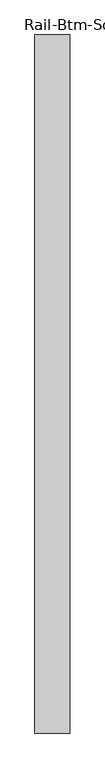
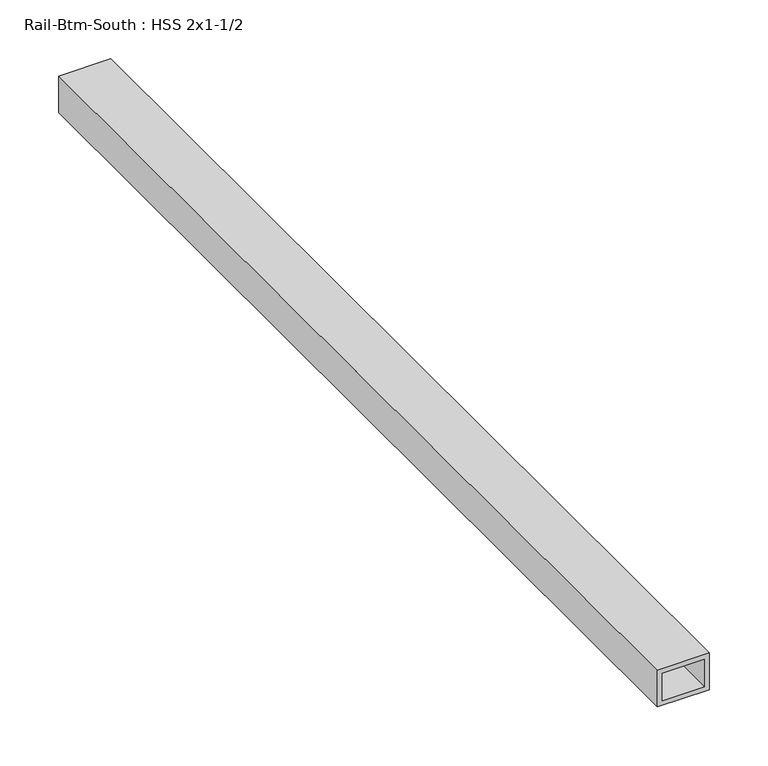
"""IFC4 building model written with IfcOpenShell, lengths in millimetres: proxy geometry, Rail-Btm-South : HSS 2x1-1/2."""

import ifcopenshell
import ifcopenshell.guid

model = None  # the IFC model being written
_history = None  # IfcOwnerHistory: only IFC2X3 demands one
_inside = {}  # id of a spatial element -> (the spatial element, [elements in it])
_under = {}  # id of a project, library or spatial element -> (it, [spatial elements below it])
_declared = {}  # id of a project -> (the project, [libraries it declares])
_typed = {}  # id of a type object -> (the type object, [elements of that type])
_made_of = {}  # id of a material, layer set ... -> (it, [elements and type objects made of it])


def new_model(schema):
    """Start an empty IFC model of exactly this schema.

    Asked for "IFC4X3", IfcOpenShell would pick the latest addendum, in which some entities
    have other attributes; the version numbers below select the first issue.
    IFC2X3 requires an IfcOwnerHistory on every rooted entity: one is made here for all.
    """
    global model, _history
    if schema == "IFC4X3":
        model = ifcopenshell.file(schema_version=(4, 3, 0, 0))
    else:
        model = ifcopenshell.file(schema=schema)
    _inside.clear()
    _under.clear()
    _declared.clear()
    _typed.clear()
    _made_of.clear()
    _history = None
    if model.schema == "IFC2X3":
        org = make("IfcOrganization", Name="unknown")
        user = make(
            "IfcPersonAndOrganization",
            ThePerson=make("IfcPerson", FamilyName="unknown"),
            TheOrganization=org,
        )
        app = make(
            "IfcApplication",
            ApplicationDeveloper=org,
            Version="unknown",
            ApplicationFullName="unknown",
            ApplicationIdentifier="unknown",
        )
        _history = make(
            "IfcOwnerHistory",
            OwningUser=user,
            OwningApplication=app,
            ChangeAction="ADDED",
            CreationDate=0,
        )
    return model


def make(cls, **values):
    """One entity of the class cls with the attributes given. An attribute that is None is left unset."""
    return model.create_entity(
        cls, **{name: value for name, value in values.items() if value is not None}
    )


def rooted(cls, **values):
    """An entity with a GlobalId (a new one), such as an element, a storey or a relation."""
    return make(cls, GlobalId=ifcopenshell.guid.new(), OwnerHistory=_history, **values)


def si_unit(unit_type, name, prefix=None):
    """IfcSIUnit, for example si_unit("LENGTHUNIT", "METRE", prefix="MILLI")."""
    return make("IfcSIUnit", UnitType=unit_type, Prefix=prefix, Name=name)


def assignment(units):
    """IfcUnitAssignment: the units of a project."""
    return None if units is None else make("IfcUnitAssignment", Units=units)


def point(xyz):
    """IfcCartesianPoint."""
    return None if xyz is None else make("IfcCartesianPoint", Coordinates=xyz)


def direction(xyz):
    """IfcDirection."""
    return None if xyz is None else make("IfcDirection", DirectionRatios=xyz)


def frame(location, z_axis=None, x_axis=None):
    """IfcAxis2Placement3D, a coordinate frame: its origin and axes. An axis left out is left unset."""
    return make(
        "IfcAxis2Placement3D",
        Location=point(location),
        Axis=direction(z_axis),
        RefDirection=direction(x_axis),
    )


def origin():
    """The frame at (0, 0, 0) with its axes left unset."""
    return frame((0.0, 0.0, 0.0))


def place(relative_to, where):
    """IfcLocalPlacement: puts the frame where relative to a parent placement (None: the world)."""
    return make(
        "IfcLocalPlacement", PlacementRelTo=relative_to, RelativePlacement=where
    )


def context(
    kind, dimensions, precision=None, world=None, true_north=None, identifier=None
):
    """IfcGeometricRepresentationContext, for example the 3D "Model" context."""
    return make(
        "IfcGeometricRepresentationContext",
        ContextIdentifier=identifier,
        ContextType=kind,
        CoordinateSpaceDimension=dimensions,
        Precision=precision,
        WorldCoordinateSystem=world,
        TrueNorth=true_north,
    )


def project(units=None, contexts=None):
    """IfcProject with its units and contexts."""
    return rooted(
        "IfcProject",
        Name="project",
        RepresentationContexts=contexts,
        UnitsInContext=assignment(units),
    )


def spatial(cls, under=None, at=None, **own):
    """A site, building, storey or space (cls), placed at a placement, below another one or the project."""
    s = rooted(cls, ObjectPlacement=at, **own)
    if under is not None:
        _under.setdefault(under.id(), (under, []))[1].append(s)
    return s


def polyline(points):
    """IfcPolyline through the points."""
    return make("IfcPolyline", Points=[point(p) for p in points])


def outline(outer, holes=None, kind="AREA"):
    """IfcArbitraryClosedProfileDef: a profile drawn as a closed curve; with holes, ...WithVoids."""
    if holes is None:
        return make("IfcArbitraryClosedProfileDef", ProfileType=kind, OuterCurve=outer)
    return make(
        "IfcArbitraryProfileDefWithVoids",
        ProfileType=kind,
        OuterCurve=outer,
        InnerCurves=holes,
    )


def extrude(swept, where, along, depth):
    """IfcExtrudedAreaSolid: the profile swept, set in the frame where, extruded along a direction by depth."""
    return make(
        "IfcExtrudedAreaSolid",
        SweptArea=swept,
        Position=where,
        ExtrudedDirection=direction(along),
        Depth=depth,
    )


def shape(context_of_items, identifier, shape_type, items):
    """IfcShapeRepresentation: the items that make up one representation, for example the "Body"."""
    return make(
        "IfcShapeRepresentation",
        ContextOfItems=context_of_items,
        RepresentationIdentifier=identifier,
        RepresentationType=shape_type,
        Items=items,
    )


def source(mapping_origin, context_of_items, identifier, shape_type, items):
    """IfcRepresentationMap: a shape defined once, which mapped items show again and again."""
    return make(
        "IfcRepresentationMap",
        MappingOrigin=mapping_origin,
        MappedRepresentation=shape(context_of_items, identifier, shape_type, items),
    )


def transform(
    local_origin,
    x_axis=None,
    y_axis=None,
    z_axis=None,
    scale=None,
    scale2=None,
    scale3=None,
    uniform=True,
):
    """IfcCartesianTransformationOperator3D, or its non-uniform kind. x_axis, y_axis, z_axis: its Axis1, 2, 3."""
    if uniform:
        return make(
            "IfcCartesianTransformationOperator3D",
            Axis1=direction(x_axis),
            Axis2=direction(y_axis),
            LocalOrigin=point(local_origin),
            Scale=scale,
            Axis3=direction(z_axis),
        )
    return make(
        "IfcCartesianTransformationOperator3DnonUniform",
        Axis1=direction(x_axis),
        Axis2=direction(y_axis),
        LocalOrigin=point(local_origin),
        Scale=scale,
        Axis3=direction(z_axis),
        Scale2=scale2,
        Scale3=scale3,
    )


def mapped(mapping_source, mapping_target):
    """IfcMappedItem: shows the shape of a source again, moved by a transform."""
    return make(
        "IfcMappedItem", MappingSource=mapping_source, MappingTarget=mapping_target
    )


def made_of(thing, what):
    """Note that an element or type object is made of a material, layer set ...; save() writes the relation."""
    if what is not None:
        _made_of.setdefault(what.id(), (what, []))[1].append(thing)
    return thing


def element(
    cls,
    number,
    at=None,
    inside=None,
    cuts=None,
    type_object=None,
    material=None,
    context=None,
    identifier="Body",
    shape_type=None,
    held_by="IfcProductDefinitionShape",
    body=None,
    shapes=None,
    **own,
):
    """One element of the class cls, such as IfcWall. Its Tag is "e" and its number.

    at: its placement. inside: the storey or other place that contains it. cuts: it is an
    opening in that element (IfcRelVoidsElement). A single representation is given by context,
    identifier, shape_type and body (its items); several are given by shapes. held_by: the class
    of the entity that holds the representations. save() writes the other relations.
    """
    e = rooted(cls, Tag="e%d" % number, ObjectPlacement=at, **own)
    if body is not None:
        shapes = [shape(context, identifier, shape_type, body)]
    if shapes is not None:
        e.Representation = make(held_by, Representations=shapes)
    if inside is not None:
        _inside.setdefault(inside.id(), (inside, []))[1].append(e)
    if cuts is not None:
        rooted(
            "IfcRelVoidsElement", RelatingBuildingElement=cuts, RelatedOpeningElement=e
        )
    if type_object is not None:
        _typed.setdefault(type_object.id(), (type_object, []))[1].append(e)
    return made_of(e, material)


def aggregate(whole, parts):
    """IfcRelAggregates: a whole, such as a stair, and the parts it consists of."""
    return rooted("IfcRelAggregates", RelatingObject=whole, RelatedObjects=parts)


def save(model, path):
    """Write the relations noted so far, then the file.

    IfcRelAggregates (storeys below a building ...), IfcRelContainedInSpatialStructure (elements
    in a storey), IfcRelDefinesByType, IfcRelAssociatesMaterial and IfcRelDeclares: one each for
    every whole, place, type object, material and project.
    """
    for whole, parts in _under.values():
        aggregate(whole, parts)
    for where, things in _inside.values():
        rooted(
            "IfcRelContainedInSpatialStructure",
            RelatedElements=things,
            RelatingStructure=where,
        )
    for kind, things in _typed.values():
        rooted("IfcRelDefinesByType", RelatedObjects=things, RelatingType=kind)
    for what, things in _made_of.values():
        rooted("IfcRelAssociatesMaterial", RelatedObjects=things, RelatingMaterial=what)
    for by, libraries in _declared.values():
        rooted("IfcRelDeclares", RelatingContext=by, RelatedDefinitions=libraries)
    model.write(path)


def rail_btm_south_hss_2x1_1_2_3b7ee801(model_context):
    return source(origin(), model_context, "Body", "SweptSolid", [
        extrude(outline(polyline([(50.8, 587416.6934739), (88.9, 587416.6934739), (88.9, 587365.8934739), (50.8, 587365.8934739), (50.8, 587416.6934739)]), holes=[polyline([(84.1375, 587411.9309739), (55.5625, 587411.9309739), (55.5625, 587370.6559739), (84.1375, 587370.6559739), (84.1375, 587411.9309739)])]), frame((0.0, -533937.9163841, 0.0), z_axis=(0.0, 1.0, 0.0), x_axis=(0.0, 0.0, 1.0)), (0.0, 0.0, 1.0), 1016.0),
    ])


if __name__ == "__main__":
    model = new_model("IFC4")
    model_context = context("Model", 3, world=origin())
    ifc_project = project(units=[si_unit("LENGTHUNIT", "METRE", prefix="MILLI")], contexts=[model_context])
    site = spatial("IfcSite", under=ifc_project)
    building = spatial("IfcBuilding", under=site)
    placement = place(None, origin())
    rail_btm_south_hss_2x1_1_2_shape = rail_btm_south_hss_2x1_1_2_3b7ee801(model_context)
    element("IfcBuildingElementProxy", 1, Name="Rail-Btm-South : HSS 2x1-1/2", ObjectType="Rail-Btm-South : HSS 2x1-1/2", at=placement, inside=building, context=model_context, shape_type="MappedRepresentation", body=[
        mapped(rail_btm_south_hss_2x1_1_2_shape, transform((0.0, 0.0, 0.0), x_axis=(1.0, 0.0, 0.0), y_axis=(0.0, 1.0, 0.0), z_axis=(0.0, 0.0, 1.0))),
    ])
    save(model, "model.ifc")

# Revit data of these elements
# Element 1 (IfcBuildingElementProxy, "Rail-Btm-South : HSS 2x1-1/2")
#   Materials on its faces: "1-1/2\"X2\" GALV. STL HSS TUBING"
# Materials
#   "1-1/2\"X2\" GALV. STL HSS TUBING": class "Generic", colour RGB 211 211 207, transparency 0, Cost = 0
